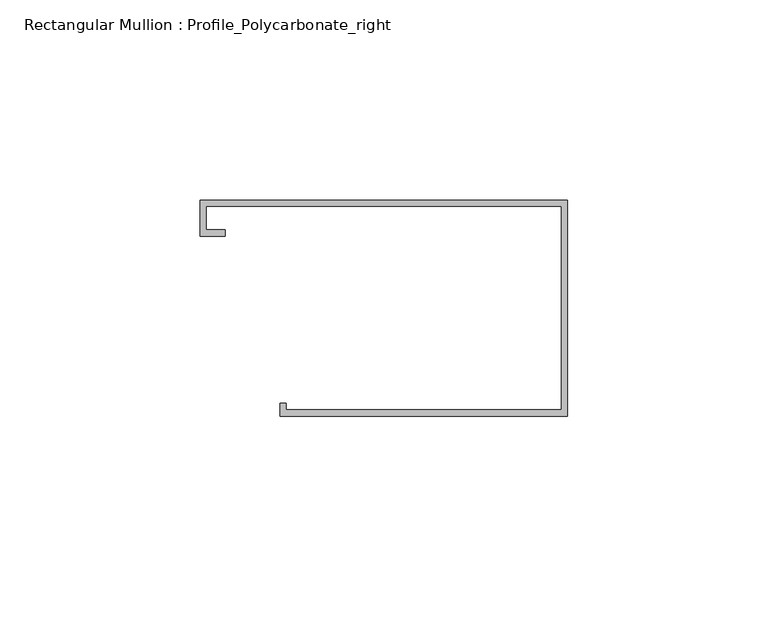
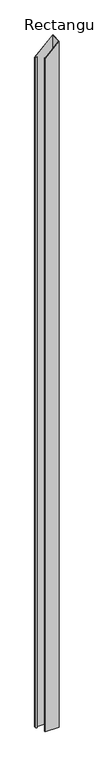
"""IFC4 building model written with IfcOpenShell, lengths in millimetres: member geometry, Rectangular Mullion : Profile_Polycarbonate_right."""

from ifc_helpers import new_model, si_unit, origin, place, context, project, spatial, faceted_brep, source, transform, mapped, element, save


def rectangular_mullion_profile_polycarbonate_right_1ad47030(model_context):
    return source(origin(), model_context, "Body", "Brep", [
        faceted_brep([(0.0, 28.984575, -3666.4630061), (0.0, -25.015825, -3666.4630061), (-71.9836, -25.015825, -3666.4630061), (-71.9836, -21.840825, -3666.4630061), (-70.3961, -21.840825, -3666.4630061), (-70.3961, -23.428325, -3666.4630061), (-1.5875, -23.428325, -3666.4630061), (-1.5875, 27.397075, -3666.4630061), (-90.4113, 27.397075, -3666.4630061), (-90.4113, 21.580475, -3666.4630061), (-85.6488, 21.580475, -3666.4630061), (-85.6488, 19.992975, -3666.4630061), (-91.9988, 19.992975, -3666.4630061), (-91.9988, 28.984575, -3666.4630061), (-91.9988, 28.984575, -88.2453421), (0.0, 28.984575, 0.0), (-91.9988, 19.992975, -88.2453421), (-85.6488, 19.992975, -82.1544157), (-85.6488, 21.580475, -82.1544157), (-90.4113, 21.580475, -86.7226105), (-90.4113, 27.397075, -86.7226105), (-1.5875, 27.397075, -1.5227316), (-1.5875, -23.428325, -1.5227316), (-70.3961, -23.428325, -67.5240104), (-70.3961, -21.840825, -67.5240104), (-71.9836, -21.840825, -69.046742), (-71.9836, -25.015825, -69.046742), (0.0, -25.015825, 0.0)], [[[0, 1, 2, 3, 4, 5, 6, 7, 8, 9, 10, 11, 12, 13]], [[14, 15, 0, 13]], [[16, 14, 13, 12]], [[17, 16, 12, 11]], [[18, 17, 11, 10]], [[19, 18, 10, 9]], [[20, 19, 9, 8]], [[21, 20, 8, 7]], [[22, 21, 7, 6]], [[23, 22, 6, 5]], [[24, 23, 5, 4]], [[25, 24, 4, 3]], [[26, 25, 3, 2]], [[27, 26, 2, 1]], [[15, 27, 1, 0]], [[15, 14, 16, 17, 18, 19, 20, 21, 22, 23, 24, 25, 26, 27]]]),
    ])


if __name__ == "__main__":
    model = new_model("IFC4")
    model_context = context("Model", 3, world=origin())
    ifc_project = project(units=[si_unit("LENGTHUNIT", "METRE", prefix="MILLI")], contexts=[model_context])
    site = spatial("IfcSite", under=ifc_project)
    building = spatial("IfcBuilding", under=site)
    placement = place(None, origin())
    rectangular_mullion_profile_polycarbonate_right_shape = rectangular_mullion_profile_polycarbonate_right_1ad47030(model_context)
    element("IfcMember", 1, ObjectType="Rectangular Mullion : Profile_Polycarbonate_right", at=placement, inside=building, context=model_context, shape_type="MappedRepresentation", body=[
        mapped(rectangular_mullion_profile_polycarbonate_right_shape, transform((0.0, 0.0, 0.0), x_axis=(1.0, 0.0, 0.0), y_axis=(0.0, 1.0, 0.0), z_axis=(0.0, 0.0, 1.0))),
    ])
    save(model, "model.ifc")

# Revit data of these elements
# Type "Rectangular Mullion : Profile_Polycarbonate_right"
#   built-in parameter 1007322 = 0.177167 (stored number, unit not read)
#   built-in parameter 1007321 = 0 (stored number, unit not read)
#   built-in parameter 1007320 = 0.00520833 (stored number, unit not read)
